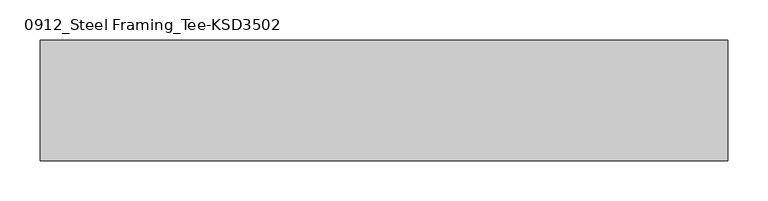
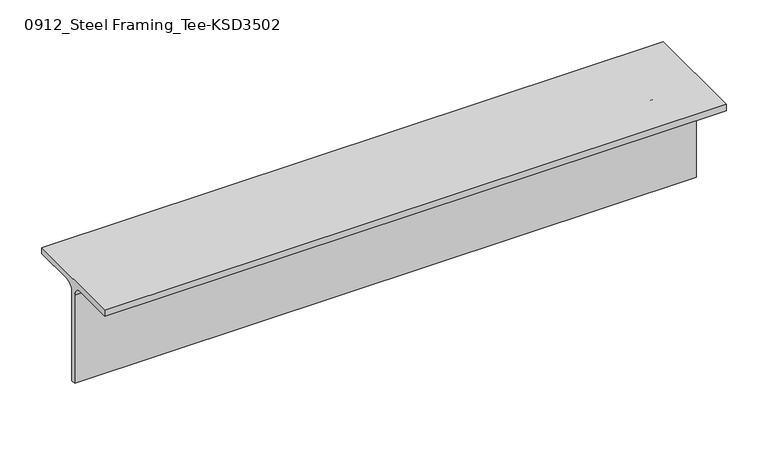
"""IFC4 building model written with IfcOpenShell, lengths in millimetres: member geometry, 0912_Steel Framing_Tee-KSD3502 : H_SB_ASB_CT-150x150x6.5x9."""

from ifc_helpers import new_model, si_unit, point, frame, frame_2d, origin, place, context, project, spatial, polyline, circle_curve, trimmed, segment, composite_curve, outline, extrude, source, transform, mapped, element, save


def member_0912_steel_framing_tee_ksd3502_0f810a09(model_context):
    return source(origin(), model_context, "Body", "SweptSolid", [
        extrude(outline(composite_curve([segment(polyline([(75.0, 75.0), (75.0, 66.0), (16.25, 66.0)]), True, "CONTINUOUS"), segment(trimmed(circle_curve(frame_2d((16.25, 53.0)), 13.0), [point((16.25, 66.0))], [point((3.25, 53.0))], True, "CARTESIAN"), True, "CONTINUOUS"), segment(polyline([(3.25, 53.0), (3.25, -75.0), (-3.25, -75.0), (-3.25, 53.0)]), True, "CONTINUOUS"), segment(trimmed(circle_curve(frame_2d((-16.25, 53.0)), 13.0), [point((-3.25, 53.0))], [point((-16.25, 66.0))], True, "CARTESIAN"), True, "CONTINUOUS"), segment(polyline([(-16.25, 66.0), (-75.0, 66.0), (-75.0, 75.0), (75.0, 75.0)]), True, "CONTINUOUS")], self_intersect=False)), frame((-500.0, 0.0, 0.0), z_axis=(1.0, 0.0, 0.0), x_axis=(0.0, 1.0, 0.0)), (0.0, 0.0, 1.0), 856.1),
    ])


if __name__ == "__main__":
    model = new_model("IFC4")
    model_context = context("Model", 3, world=origin())
    ifc_project = project(units=[si_unit("LENGTHUNIT", "METRE", prefix="MILLI")], contexts=[model_context])
    site = spatial("IfcSite", under=ifc_project)
    building = spatial("IfcBuilding", under=site)
    placement = place(None, origin())
    member_0912_steel_framing_tee_ksd3502_shape = member_0912_steel_framing_tee_ksd3502_0f810a09(model_context)
    element("IfcMember", 1, ObjectType="0912_Steel Framing_Tee-KSD3502 : H_SB_ASB_CT-150x150x6.5x9", at=placement, inside=building, context=model_context, shape_type="MappedRepresentation", body=[
        mapped(member_0912_steel_framing_tee_ksd3502_shape, transform((0.0, 0.0, 0.0), x_axis=(1.0, 0.0, 0.0), y_axis=(0.0, 1.0, 0.0), z_axis=(0.0, 0.0, 1.0))),
    ])
    save(model, "model.ifc")

# Revit data of these elements
# Type "0912_Steel Framing_Tee-KSD3502 : H_SB_ASB_CT-150x150x6.5x9"
#   H_WM Code_1 = "S01AA003-00001 | Main Steel Structure Fabrication Work | Shelter/Building | Light Steel - Standard (30KG/M>Weight) | Material: (   )"
#   H_WM Code_2 = "S03AA029-00001 | Main Steel Structure Erection Work | Shelter/Building | Light Steel (30KG/M>Weight) | Material: (   )"
#   H_WM Code_3 = "S01AA010-00001 | Main Steel Structure Fabrication Work | Shelter/Building | Steel Painting/Coating | for Non-Fireproofed Steel Surface, Surface Preparation, Primer, Second & Final Coat | Material: (   )"
#   H_Q'ty Cal Type Tag = "SB-Q2"
#   Width = 15.0 cm
#   Web Thickness = 0.65 cm
#   Web Fillet = 1.3 cm
#   Section Area = 23.39 cm²
#   Perimeter = 0.60 m²/m
#   Nominal Weight = 18.40 kgf/m
#   Height = 15.0 cm
#   Flange Thickness = 0.9 cm
#   Centroid Vertical = 7.5 cm
#   Centroid Horizontal = 7.5 cm
#   Length [instance default] = 1.5000 m
#   Structural Material [instance default] = Steel, 45-345
#   Warping Constant = (empty or 0)
#   Torsional Moment of Inertia = 0
#   Section Name Key = ""
#   Plastic Modulus weak axis = 0
#   Plastic Modulus strong axis = 0
#   Moment of Inertia weak axis = 0
#   Moment of Inertia strong axis = 0
#   Elastic Modulus weak axis = 0
#   Elastic Modulus strong axis = 0
#   Bolt Spacing = 0
#   Assembly Code = ""
# Element 1 (IfcMember, "0912_Steel Framing_Tee-KSD3502 : H_SB_ASB_CT-150x150x6.5x9")
#   Structural Material = none
# Materials
#   "Steel, 45-345": class "Metal", colour RGB 189 187 185, transparency 0, Description = "Steel 345 MPa", Cost = 0
